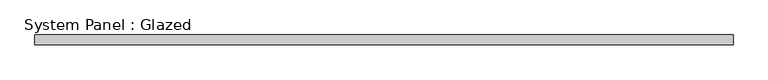
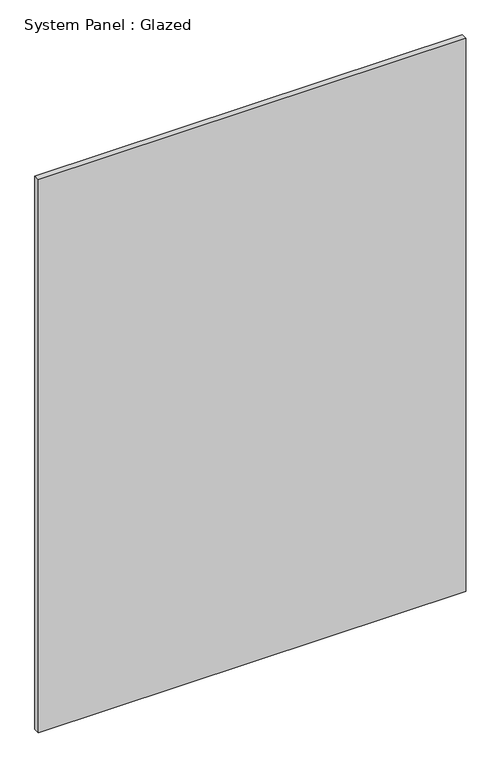
"""IFC4 building model written with IfcOpenShell, lengths in millimetres: plate geometry, System Panel : Glazed."""

from ifc_helpers import new_model, si_unit, origin, origin_with_axes, place, context, project, spatial, polyline, outline, extrude, source, transform, mapped, element, save


def system_panel_glazed_491828d4(model_context):
    return source(origin(), model_context, "Body", "SweptSolid", [
        extrude(outline(polyline([(890.0000002, 24.5), (-890.0000002, 24.5), (-890.0000002, 49.5), (890.0000002, 49.5), (890.0000002, 24.5)])), origin_with_axes(), (0.0, 0.0, 1.0), 2435.0),
    ])


if __name__ == "__main__":
    model = new_model("IFC4")
    model_context = context("Model", 3, world=origin())
    ifc_project = project(units=[si_unit("LENGTHUNIT", "METRE", prefix="MILLI")], contexts=[model_context])
    site = spatial("IfcSite", under=ifc_project)
    building = spatial("IfcBuilding", under=site)
    placement = place(None, origin())
    system_panel_glazed_shape = system_panel_glazed_491828d4(model_context)
    element("IfcPlate", 1, ObjectType="System Panel : Glazed", at=placement, inside=building, context=model_context, shape_type="MappedRepresentation", body=[
        mapped(system_panel_glazed_shape, transform((0.0, 0.0, 0.0), x_axis=(1.0, 0.0, 0.0), y_axis=(0.0, 1.0, 0.0), z_axis=(0.0, 0.0, 1.0))),
    ])
    save(model, "model.ifc")

# Revit data of these elements
# Element 1 (IfcPlate, "System Panel : Glazed")
#   Materials on its faces: "Glass"
# Materials
#   "Glass": class "Glass", colour RGB 218 227 224, transparency 0.85, Description = "Soda Lime Glass", Cost = 0
